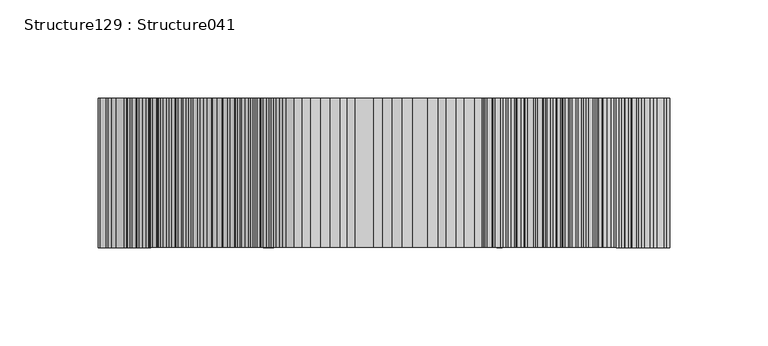
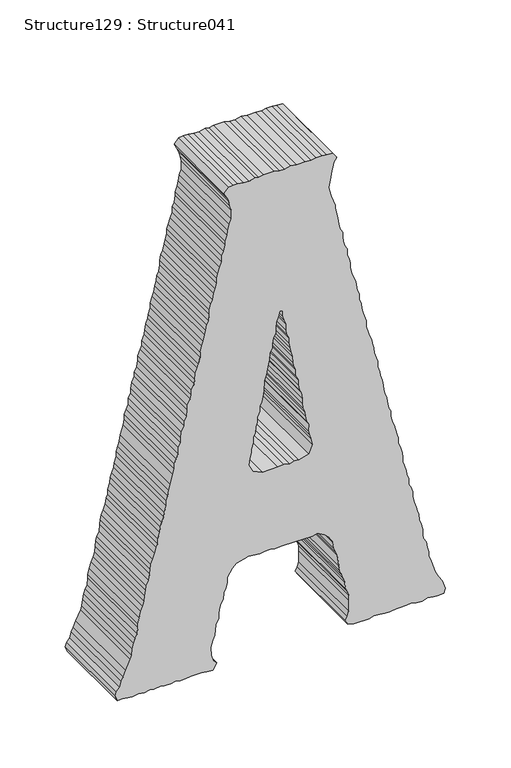
"""IFC4 building model written with IfcOpenShell, lengths in millimetres: proxy geometry, Structure129 : Structure041."""

from ifc_helpers import new_model, si_unit, frame, origin, place, context, project, spatial, polyline, outline, extrude, source, transform, mapped, element, save


def structure129_structure041_3d3b70dd(model_context):
    return source(origin(), model_context, "Body", "SweptSolid", [
        extrude(outline(polyline([(3818.8310229, -41916.3907537), (3814.7296538, -41916.3907537), (3811.2043377, -41917.5717426), (3805.9476534, -41919.8903961), (3801.8462843, -41919.8903961), (3795.960595, -41920.4921228), (3791.8865042, -41922.8316362), (3787.7867397, -41922.8316362), (3783.0868532, -41925.193614), (3777.8285642, -41925.7728762), (3773.11905, -41925.7728762), (3769.6274306, -41928.1139942), (3763.759392, -41928.1139942), (3759.6596275, -41929.8742453), (3755.559863, -41931.6344964), (3750.8583719, -41931.6344964), (3746.1745313, -41932.7930209), (3737.400554, -41935.1341388), (3732.1149867, -41936.3151278), (3727.4311462, -41937.4736522), (3723.3313817, -41938.6546411), (3718.6571688, -41938.6546411), (3713.3555556, -41940.4148922), (3709.2718371, -41941.0166189), (3704.5879966, -41942.7560102), (3701.0723082, -41943.9369991), (3695.786741, -41944.5162613), (3690.512406, -41946.2765125), (3685.8285655, -41946.2765125), (3682.8857208, -41947.4575014), (3677.6274319, -41948.6176304), (3672.9435914, -41950.3778816), (3668.8261762, -41952.1381327), (3664.1423357, -41952.7173949), (3660.0682449, -41953.2966571), (3654.1841602, -41953.8983838), (3650.1004418, -41956.2395018), (3645.9830266, -41956.8412285), (3641.2991861, -41957.3980262), (3636.0408972, -41957.9772884), (3631.915459, -41959.1582774), (3627.8397636, -41960.9185285), (3622.555801, -41962.6787796), (3617.2718384, -41963.8613731), (3613.772196, -41963.8613731), (3607.8961343, -41964.4406354), (3604.3964919, -41966.2008865), (3600.2967274, -41967.3594109), (3595.5872132, -41968.5403998), (3589.7544759, -41969.1196621), (3586.2115092, -41970.300651), (3577.4535778, -41974.4020201), (3572.1423369, -41976.7415334), (3568.6426945, -41978.5033892), (3563.366755, -41979.6619136), (3560.441561, -41982.6031536), (3556.3417965, -41983.7841425), (3551.6675836, -41982.001427), (3551.6675836, -41977.3432601), (3551.0658569, -41972.6417689), (3550.4833855, -41968.5403998), (3551.6675836, -41963.2805063), (3550.4833855, -41957.9772884), (3551.6675836, -41953.2966571), (3551.0658569, -41949.7761549), (3551.6675836, -41943.9369991), (3551.0658569, -41940.4148922), (3551.0658569, -41934.5773411), (3551.6675836, -41930.4535075), (3551.0658569, -41926.353743), (3551.0658569, -41921.6506473), (3551.6675836, -41916.9924804), (3551.6675836, -41907.6103579), (3551.0658569, -41902.9297266), (3550.4833855, -41897.6265088), (3556.3417965, -41894.1268664), (3559.2669905, -41897.0472465), (3565.1254015, -41898.8074977), (3572.7440636, -41899.3867599), (3578.6104977, -41897.6265088), (3582.7102621, -41895.8871175), (3587.3860796, -41895.3078553), (3592.0955938, -41894.728593), (3596.7698067, -41892.3666152), (3601.4536473, -41892.3666152), (3604.9709403, -41891.787353), (3610.2292293, -41890.6063641), (3613.772196, -41888.2652461), (3619.6145609, -41887.6859839), (3622.555801, -41885.9257328), (3627.8397636, -41884.7447439), (3633.0980525, -41884.7447439), (3639.5405396, -41880.0641126), (3643.0578326, -41876.5436103), (3644.8245022, -41869.5234656), (3645.9830266, -41866.0013588), (3645.4262289, -41860.1413431), (3644.8245022, -41856.039974), (3645.4262289, -41851.3593427), (3645.9830266, -41846.6578516), (3644.8245022, -41842.5789469), (3645.4262289, -41837.2757291), (3645.4262289, -41824.9956909), (3644.8245022, -41819.1340706), (3644.8245022, -41809.7519482), (3645.9830266, -41805.0713168), (3642.4833842, -41798.6304344), (3638.9580681, -41794.5082054), (3633.0980525, -41791.6102897), (3627.2396415, -41790.4293008), (3622.555801, -41788.6690497), (3619.6145609, -41787.4880608), (3609.0723094, -41786.3070719), (3604.3964919, -41785.1485474), (3600.2967274, -41783.9884184), (3596.1953583, -41782.2281672), (3592.0955938, -41781.0471783), (3586.2115092, -41780.4679161), (3582.7102621, -41778.6852005), (3578.6104977, -41777.5266761), (3573.9266571, -41777.5266761), (3563.9412034, -41777.5266761), (3559.2669905, -41778.6852005), (3555.7416744, -41780.4679161), (3551.6675836, -41778.1059383), (3550.4833855, -41772.8460448), (3550.4833855, -41759.3625532), (3551.6675836, -41755.2627887), (3551.0658569, -41749.9804307), (3550.4833855, -41745.2997994), (3550.4833855, -41741.2000349), (3551.0658569, -41735.3384147), (3551.0658569, -41731.25951), (3551.6675836, -41726.5580189), (3551.6675836, -41722.4566498), (3550.4833855, -41717.7551586), (3550.4833855, -41712.4952651), (3551.6675836, -41707.8146338), (3551.0658569, -41702.5114159), (3550.4833855, -41699.0117735), (3551.0658569, -41693.1726177), (3555.1848766, -41691.9916288), (3560.441561, -41693.75188), (3563.366755, -41694.9104044), (3568.6426945, -41698.4325113), (3572.1423369, -41700.1927624), (3576.2693797, -41701.9530135), (3586.2115092, -41704.8733937), (3590.3289243, -41706.6336448), (3594.4286888, -41706.6336448), (3599.1125293, -41707.8146338), (3604.3964919, -41708.9956227), (3608.4705827, -41711.3142762), (3612.5976255, -41711.8935384), (3617.2718384, -41711.8935384), (3622.555801, -41713.0745273), (3627.2396415, -41714.8347784), (3632.5155811, -41715.4365051), (3636.0408972, -41716.5950296), (3640.114988, -41717.7551586), (3645.4262289, -41719.5154097), (3650.6845178, -41720.6963986), (3655.3587307, -41720.6963986), (3659.4584952, -41721.8773876), (3663.5598643, -41724.2169009), (3668.8261762, -41724.2169009), (3673.5276674, -41725.9562922), (3677.0449605, -41726.5580189), (3682.8857208, -41728.31827), (3686.4030139, -41729.4767944), (3691.0868544, -41729.4767944), (3695.2122926, -41730.0785211), (3699.8881101, -41731.25951), (3705.7545441, -41733.5781635), (3710.4560353, -41733.5781635), (3714.5301261, -41734.7591524), (3718.0554422, -41735.9401414), (3723.3313817, -41737.0986658), (3727.4311462, -41738.8589169), (3732.7167134, -41740.019046), (3737.9750024, -41740.019046), (3740.9162424, -41741.7792971), (3745.6000829, -41742.960286), (3751.4424479, -41743.5395482), (3756.1423345, -41745.2997994), (3759.6596275, -41746.4807883), (3764.3611187, -41747.0600505), (3769.0176809, -41747.6409173), (3774.3032481, -41749.4011685), (3777.8285642, -41749.9804307), (3783.0868532, -41751.7406818), (3788.3611881, -41751.7406818), (3791.8865042, -41752.9216707), (3797.1463977, -41754.661062), (3801.8462843, -41755.2627887), (3806.5317294, -41756.4213131), (3810.0474179, -41757.0230398), (3815.3313805, -41759.3625532), (3820.015221, -41760.5435421), (3824.1149855, -41761.724531), (3829.374879, -41761.724531), (3837.6000817, -41764.6449112), (3842.8583706, -41765.8034356), (3846.9757858, -41766.4051623), (3851.6612309, -41768.1654134), (3856.9179152, -41768.1654134), (3861.0192843, -41769.9048047), (3866.3032469, -41770.4840669), (3869.8189354, -41771.0857936), (3873.9203044, -41772.8460448), (3878.5784713, -41774.6062959), (3883.8881076, -41775.7872848), (3888.5623205, -41775.7872848), (3892.6636896, -41776.9458092), (3897.3475301, -41778.6852005), (3902.6314927, -41778.6852005), (3906.1487857, -41781.0471783), (3910.8310217, -41782.2281672), (3916.0909152, -41782.8074295), (3919.6066036, -41782.8074295), (3924.2888396, -41785.1485474), (3928.9919353, -41786.3070719), (3934.2758979, -41786.9087986), (3938.9517154, -41788.067323), (3944.235678, -41789.2483119), (3947.1496398, -41789.2483119), (3956.5349715, -41792.7479543), (3961.794865, -41793.9289432), (3965.8930249, -41795.1099321), (3974.7055128, -41793.349681), (3979.9621971, -41792.1686921), (3983.4794902, -41791.6102897), (3987.5792547, -41790.4293008), (3991.6806238, -41788.067323), (3996.390138, -41791.6102897), (3996.9645864, -41796.8701833), (3997.5486624, -41800.9490879), (3997.5486624, -41806.2523058), (3996.390138, -41810.3312104), (3996.9645864, -41815.6135684), (3996.9645864, -41823.2129753), (3997.5486624, -41828.5161931), (3996.390138, -41833.7760867), (3996.390138, -41838.456718), (3997.5486624, -41843.1582092), (3997.5486624, -41852.5194718), (3996.9645864, -41856.6417007), (3997.5486624, -41860.1413431), (3996.390138, -41865.4220965), (3996.390138, -41870.1027278), (3997.5486624, -41875.3626214), (3997.5486624, -41879.4848503), (3996.9645864, -41883.5862194), (3992.2614906, -41887.6859839), (3987.5792547, -41885.3464706), (3984.0635662, -41883.5862194), (3979.3781211, -41882.4052305), (3974.7055128, -41881.2451015), (3966.5043792, -41881.2451015), (3962.3757319, -41882.9844927), (3957.1190475, -41884.1654816), (3952.435207, -41884.7447439), (3947.7337158, -41886.504995), (3944.235678, -41886.504995), (3938.3499888, -41887.6859839), (3934.8503464, -41889.4478396), (3929.5904528, -41889.4478396), (3924.8905662, -41891.1856263), (3919.6066036, -41892.9458774), (3915.5068392, -41894.1268664), (3910.8310217, -41894.1268664), (3906.1487857, -41895.3078553), (3902.6314927, -41896.4888442), (3896.763454, -41897.6265088), (3893.822214, -41899.3867599), (3888.5623205, -41900.5677488), (3884.4609514, -41900.5677488), (3878.5784713, -41901.1694755), (3875.0772243, -41902.9297266), (3870.4030114, -41903.5089888), (3866.3032469, -41904.6691179), (3861.0192843, -41905.8501068), (3856.9179152, -41907.0086312), (3851.6612309, -41908.7688824), (3846.9757858, -41908.7688824), (3841.6741725, -41910.5291335), (3838.1761347, -41911.1308602), (3833.4730389, -41912.8702515), (3828.2163546, -41913.4495137), (3824.1149855, -41914.0512404), (3818.8310229, -41916.3907537)]), holes=[polyline([(3720.4158154, -41853.7004607), (3723.9154578, -41861.9015943), (3730.9323932, -41865.4220965), (3736.7988273, -41864.2411076), (3741.5003184, -41863.0825832), (3744.9999608, -41863.0825832), (3750.3015741, -41861.2998676), (3755.559863, -41861.2998676), (3759.0595054, -41859.5620809), (3764.3611187, -41858.9812141), (3768.4432325, -41857.8002252), (3773.11905, -41857.8002252), (3777.8285642, -41855.4607118), (3783.0868532, -41855.4607118), (3786.0280932, -41853.7004607), (3790.7039107, -41853.098734), (3795.4037973, -41851.9610694), (3804.7730829, -41851.3593427), (3810.0474179, -41849.5990916), (3814.7296538, -41849.0198294), (3818.8310229, -41847.8388405), (3822.932392, -41847.2595782), (3828.790803, -41846.6578516), (3833.4730389, -41844.3391981), (3836.9919366, -41844.3391981), (3842.2758992, -41843.7374714), (3845.8012153, -41841.397958), (3851.0595042, -41841.397958), (3855.7353217, -41840.8186958), (3860.4432313, -41839.0359802), (3865.1190488, -41837.8774558), (3864.5446004, -41836.1380645), (3860.4432313, -41836.1380645), (3856.3161885, -41834.9570756), (3851.6612309, -41833.1968244), (3846.3772683, -41833.1968244), (3842.2758992, -41832.5950978), (3837.6000817, -41830.2555844), (3832.8921721, -41830.2555844), (3828.790803, -41829.6763222), (3824.1149855, -41828.5161931), (3819.4150989, -41827.3352042), (3813.5743386, -41826.755942), (3810.0474179, -41826.1542153), (3805.9476534, -41824.3939642), (3800.6717138, -41824.3939642), (3795.4037973, -41822.0544508), (3790.7039107, -41822.0544508), (3786.0280932, -41820.8943218), (3782.5027771, -41819.1340706), (3777.2444882, -41818.5548084), (3772.5606477, -41818.5548084), (3767.8607611, -41817.9530817), (3763.759392, -41816.1928306), (3759.6596275, -41815.6135684), (3754.9854146, -41815.0118417), (3750.8583719, -41812.6931882), (3744.9999608, -41813.2724504), (3740.9162424, -41812.0914615), (3736.7988273, -41810.9329371), (3730.9323932, -41809.7519482), (3723.3313817, -41812.6931882), (3720.4158154, -41821.473584), (3720.9726131, -41825.5749531), (3719.8140887, -41829.6763222), (3720.9726131, -41834.9570756), (3720.4158154, -41840.2169691), (3720.4158154, -41853.7004607)])]), frame((0.0, 247945.1599557, 0.0), z_axis=(0.0, 1.0, 0.0), x_axis=(0.0, 0.0, 1.0)), (0.0, 0.0, 1.0), 76.2),
    ])


if __name__ == "__main__":
    model = new_model("IFC4")
    model_context = context("Model", 3, world=origin())
    ifc_project = project(units=[si_unit("LENGTHUNIT", "METRE", prefix="MILLI")], contexts=[model_context])
    site = spatial("IfcSite", under=ifc_project)
    building = spatial("IfcBuilding", under=site)
    placement = place(None, origin())
    structure129_structure041_shape = structure129_structure041_3d3b70dd(model_context)
    element("IfcBuildingElementProxy", 1, Name="Structure129 : Structure041", ObjectType="Structure129 : Structure041", at=placement, inside=building, context=model_context, shape_type="MappedRepresentation", body=[
        mapped(structure129_structure041_shape, transform((0.0, 0.0, 0.0), x_axis=(1.0, 0.0, 0.0), y_axis=(0.0, 1.0, 0.0), z_axis=(0.0, 0.0, 1.0))),
    ])
    save(model, "model.ifc")

# Revit data of these elements
# Type "Structure129 : Structure041"
#   NameOverride = "Structure041"
# Element 1 (IfcBuildingElementProxy, "Structure129 : Structure041")
#   Materials on its faces: "BRUSHED ALUM. LETTERING"
# Materials
#   "BRUSHED ALUM. LETTERING": class "Unassigned", colour RGB 169 181 186, transparency 0, Cost = 0
